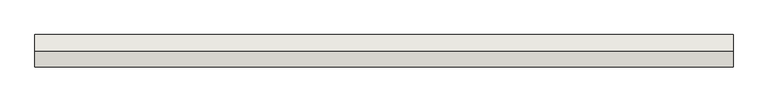
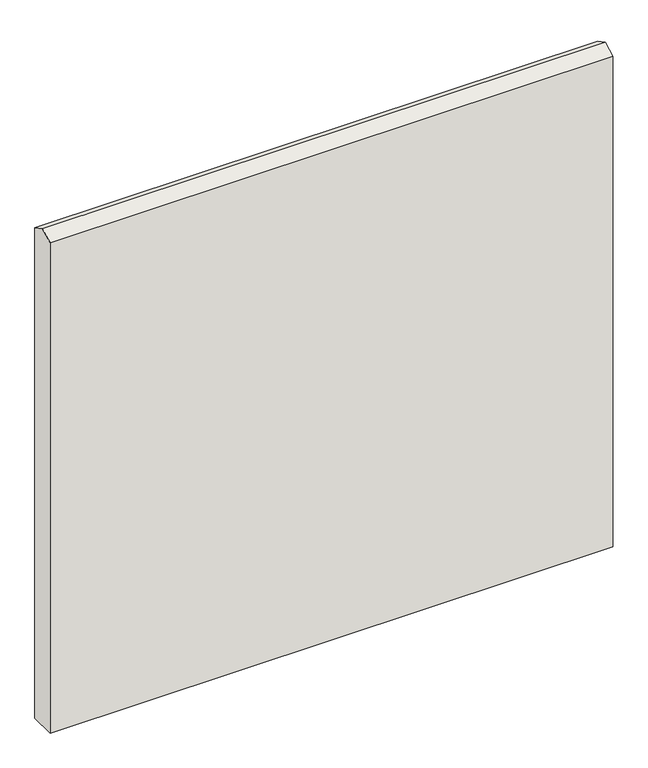
"""IFC4 building model written with IfcOpenShell, lengths in millimetres: wall geometry, Holzwand."""

from ifc_helpers import new_model, si_unit, frame, origin, place, context, project, spatial, polyline, outline, extrude, source, transform, mapped, element, save


def wall_3d93774c(model_context):
    return source(origin(), model_context, "Body", "SweptSolid", [
        extrude(outline(polyline([(100.0, 4011.6781465), (200.0, 3960.7256015), (200.0, 0.0), (0.0, 0.0), (0.0, 3960.7256015), (100.0, 4011.6781465)])), frame((0.0, 0.0, 0.0), z_axis=(1.0, 0.0, 0.0), x_axis=(0.0, 1.0, 0.0)), (0.0, 0.0, 1.0), 4297.8619019),
    ])


if __name__ == "__main__":
    model = new_model("IFC4")
    model_context = context("Model", 3, world=origin())
    ifc_project = project(units=[si_unit("LENGTHUNIT", "METRE", prefix="MILLI")], contexts=[model_context])
    site = spatial("IfcSite", under=ifc_project)
    building = spatial("IfcBuilding", under=site)
    placement = place(None, origin())
    wall_shape = wall_3d93774c(model_context)
    element("IfcWall", 1, ObjectType="Holzwand", at=placement, inside=building, context=model_context, shape_type="MappedRepresentation", body=[
        mapped(wall_shape, transform((0.0, 0.0, 0.0), x_axis=(1.0, 0.0, 0.0), y_axis=(0.0, 1.0, 0.0), z_axis=(0.0, 0.0, 1.0))),
    ])
    save(model, "model.ifc")

# Revit data of these elements
# Element 1 (IfcWall, "Holzwand")
#   Materials on its faces: "holzschalung"
# Materials
#   "holzschalung": class "Unassigned", colour RGB 128 128 128, transparency 0
